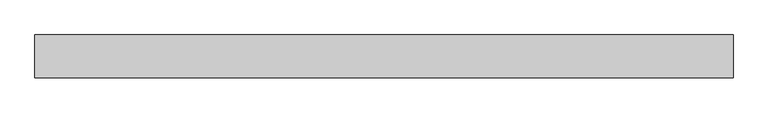
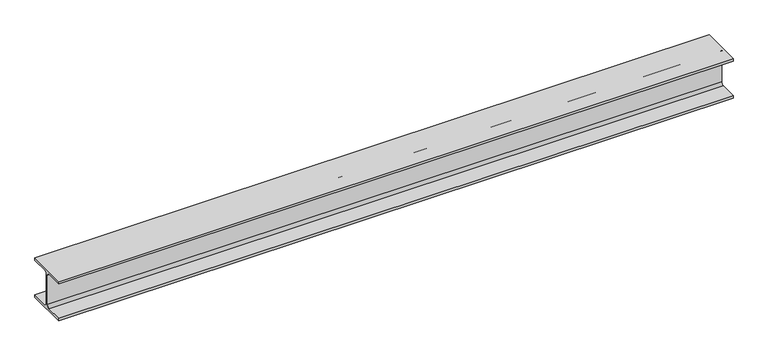
"""IFC4 building model written with IfcOpenShell, lengths in millimetres: beam geometry, 0912_Steel Framing_H-KSD3502 : H_SB_ASB_H-200x200x8x12."""

from ifc_helpers import new_model, si_unit, point, frame, frame_2d, origin, place, context, project, spatial, polyline, circle_curve, trimmed, segment, composite_curve, outline, extrude, source, transform, mapped, element, save


def beam_25fc42c0(model_context):
    return source(origin(), model_context, "Body", "SweptSolid", [
        extrude(outline(composite_curve([segment(polyline([(100.0, -88.0), (100.0, -100.0), (-100.0, -100.0), (-100.0, -88.0), (-17.0, -88.0)]), True, "CONTINUOUS"), segment(trimmed(circle_curve(frame_2d((-17.0, -75.0)), 13.0), [point((-17.0, -88.0))], [point((-4.0, -75.0))], True, "CARTESIAN"), True, "CONTINUOUS"), segment(polyline([(-4.0, -75.0), (-4.0, 75.0)]), True, "CONTINUOUS"), segment(trimmed(circle_curve(frame_2d((-17.0, 75.0)), 13.0), [point((-4.0, 75.0))], [point((-17.0, 88.0))], True, "CARTESIAN"), True, "CONTINUOUS"), segment(polyline([(-17.0, 88.0), (-100.0, 88.0), (-100.0, 100.0), (100.0, 100.0), (100.0, 88.0), (17.0, 88.0)]), True, "CONTINUOUS"), segment(trimmed(circle_curve(frame_2d((17.0, 75.0)), 13.0), [point((17.0, 88.0))], [point((4.0, 75.0))], True, "CARTESIAN"), True, "CONTINUOUS"), segment(polyline([(4.0, 75.0), (4.0, -75.0)]), True, "CONTINUOUS"), segment(trimmed(circle_curve(frame_2d((17.0, -75.0)), 13.0), [point((4.0, -75.0))], [point((17.0, -88.0))], True, "CARTESIAN"), True, "CONTINUOUS"), segment(polyline([(17.0, -88.0), (100.0, -88.0)]), True, "CONTINUOUS")], self_intersect=False)), frame((-1674.0143894, 0.0, 0.0), z_axis=(1.0, 0.0, 0.0), x_axis=(0.0, 1.0, 0.0)), (0.0, 0.0, 1.0), 3242.0146865),
    ])


if __name__ == "__main__":
    model = new_model("IFC4")
    model_context = context("Model", 3, world=origin())
    ifc_project = project(units=[si_unit("LENGTHUNIT", "METRE", prefix="MILLI")], contexts=[model_context])
    site = spatial("IfcSite", under=ifc_project)
    building = spatial("IfcBuilding", under=site)
    placement = place(None, origin())
    beam_shape = beam_25fc42c0(model_context)
    element("IfcBeam", 1, ObjectType="0912_Steel Framing_H-KSD3502 : H_SB_ASB_H-200x200x8x12", at=placement, inside=building, context=model_context, shape_type="MappedRepresentation", body=[
        mapped(beam_shape, transform((0.0, 0.0, 0.0), x_axis=(1.0, 0.0, 0.0), y_axis=(0.0, 1.0, 0.0), z_axis=(0.0, 0.0, 1.0))),
    ])
    save(model, "model.ifc")

# Revit data of these elements
# Type "0912_Steel Framing_H-KSD3502 : H_SB_ASB_H-200x200x8x12"
#   H_WM Code_1 = "S01AA002-00001 | Main Steel Structure Fabrication Work | Shelter/Building | Medium Steel - Standard (90KG/M>Weight≥30KG/M) | Material: (   )"
#   H_WM Code_2 = "S03AA028-00001 | Main Steel Structure Erection Work | Shelter/Building | Medium Steel (90KG/M>Weight≥30KG/M) | Material: (   )"
#   H_WM Code_3 = "S01AA010-00001 | Main Steel Structure Fabrication Work | Shelter/Building | Steel Painting/Coating | for Non-Fireproofed Steel Surface, Surface Preparation, Primer, Second & Final Coat | Material: (   )"
#   H_Q'ty Cal Type Tag = "SB-Q2"
#   Width = 20.0 cm
#   Web Thickness = 0.8 cm
#   Web Fillet = 1.3 cm
#   Warping Constant = 141000.0 cm⁶
#   W = 0
#   Torsional Moment of Inertia = 26.2485 cm⁴
#   Section Area = 63.53 cm²
#   Plastic Modulus weak axis = 244.0 cm³
#   Plastic Modulus strong axis = 525.0 cm³
#   Perimeter = 1.16 m²/m
#   Nominal Weight = 49.90 kgf/m
#   Moment of Inertia weak axis = 1600.00 cm⁴
#   Moment of Inertia strong axis = 4720.00 cm⁴
#   Height = 20.0 cm
#   Flange Thickness = 1.2 cm
#   Elastic Modulus weak axis = 160.0 cm³
#   Elastic Modulus strong axis = 472.0 cm³
#   Centroid Vertical = 10.0 cm
#   Centroid Horizontal = 10.0 cm
#   Ix = 47200000
#   Length [instance default] = 1.5240 m
#   Zx = 525000
#   b = 0.2000 m
#   h = 0.2000 m
#   r = 0.0130 m
#   s = 0.0080 m
#   t = 0.0120 m
#   A = 0.006353 m²
#   Structural Material [instance default] = Steel, 45-345
#   Assembly Code = ""
# Element 1 (IfcBeam, "0912_Steel Framing_H-KSD3502 : H_SB_ASB_H-200x200x8x12")
#   Structural Material = none
# Materials
#   "Steel, 45-345": class "Metal", colour RGB 189 187 185, transparency 0, Description = "Steel 345 MPa", Cost = 0
